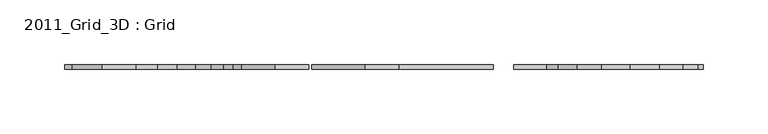
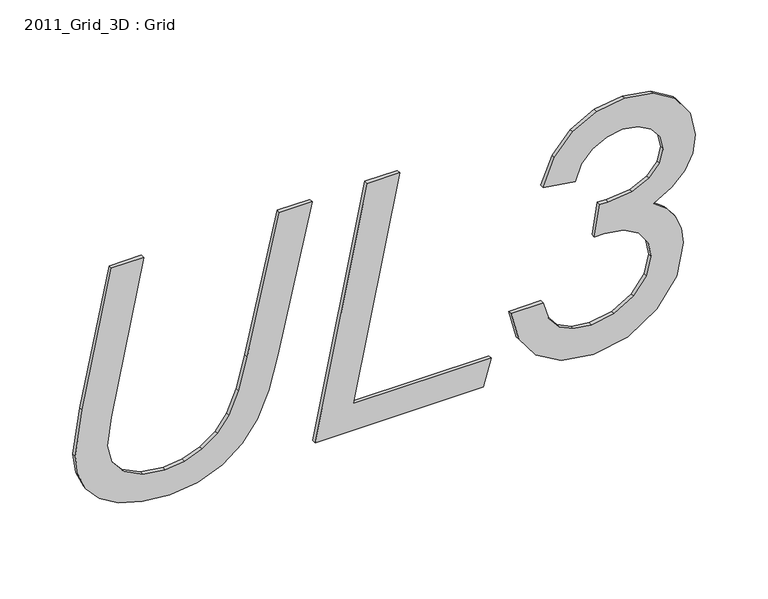
"""IFC4 building model written with IfcOpenShell, lengths in millimetres: proxy geometry, 2011_Grid_3D : Grid."""

import ifcopenshell
import ifcopenshell.guid

model = None  # the IFC model being written
_history = None  # IfcOwnerHistory: only IFC2X3 demands one
_inside = {}  # id of a spatial element -> (the spatial element, [elements in it])
_under = {}  # id of a project, library or spatial element -> (it, [spatial elements below it])
_declared = {}  # id of a project -> (the project, [libraries it declares])
_typed = {}  # id of a type object -> (the type object, [elements of that type])
_made_of = {}  # id of a material, layer set ... -> (it, [elements and type objects made of it])


def new_model(schema):
    """Start an empty IFC model of exactly this schema.

    Asked for "IFC4X3", IfcOpenShell would pick the latest addendum, in which some entities
    have other attributes; the version numbers below select the first issue.
    IFC2X3 requires an IfcOwnerHistory on every rooted entity: one is made here for all.
    """
    global model, _history
    if schema == "IFC4X3":
        model = ifcopenshell.file(schema_version=(4, 3, 0, 0))
    else:
        model = ifcopenshell.file(schema=schema)
    _inside.clear()
    _under.clear()
    _declared.clear()
    _typed.clear()
    _made_of.clear()
    _history = None
    if model.schema == "IFC2X3":
        org = make("IfcOrganization", Name="unknown")
        user = make(
            "IfcPersonAndOrganization",
            ThePerson=make("IfcPerson", FamilyName="unknown"),
            TheOrganization=org,
        )
        app = make(
            "IfcApplication",
            ApplicationDeveloper=org,
            Version="unknown",
            ApplicationFullName="unknown",
            ApplicationIdentifier="unknown",
        )
        _history = make(
            "IfcOwnerHistory",
            OwningUser=user,
            OwningApplication=app,
            ChangeAction="ADDED",
            CreationDate=0,
        )
    return model


def make(cls, **values):
    """One entity of the class cls with the attributes given. An attribute that is None is left unset."""
    return model.create_entity(
        cls, **{name: value for name, value in values.items() if value is not None}
    )


def rooted(cls, **values):
    """An entity with a GlobalId (a new one), such as an element, a storey or a relation."""
    return make(cls, GlobalId=ifcopenshell.guid.new(), OwnerHistory=_history, **values)


def si_unit(unit_type, name, prefix=None):
    """IfcSIUnit, for example si_unit("LENGTHUNIT", "METRE", prefix="MILLI")."""
    return make("IfcSIUnit", UnitType=unit_type, Prefix=prefix, Name=name)


def assignment(units):
    """IfcUnitAssignment: the units of a project."""
    return None if units is None else make("IfcUnitAssignment", Units=units)


def point(xyz):
    """IfcCartesianPoint."""
    return None if xyz is None else make("IfcCartesianPoint", Coordinates=xyz)


def direction(xyz):
    """IfcDirection."""
    return None if xyz is None else make("IfcDirection", DirectionRatios=xyz)


def frame(location, z_axis=None, x_axis=None):
    """IfcAxis2Placement3D, a coordinate frame: its origin and axes. An axis left out is left unset."""
    return make(
        "IfcAxis2Placement3D",
        Location=point(location),
        Axis=direction(z_axis),
        RefDirection=direction(x_axis),
    )


def origin():
    """The frame at (0, 0, 0) with its axes left unset."""
    return frame((0.0, 0.0, 0.0))


def place(relative_to, where):
    """IfcLocalPlacement: puts the frame where relative to a parent placement (None: the world)."""
    return make(
        "IfcLocalPlacement", PlacementRelTo=relative_to, RelativePlacement=where
    )


def context(
    kind, dimensions, precision=None, world=None, true_north=None, identifier=None
):
    """IfcGeometricRepresentationContext, for example the 3D "Model" context."""
    return make(
        "IfcGeometricRepresentationContext",
        ContextIdentifier=identifier,
        ContextType=kind,
        CoordinateSpaceDimension=dimensions,
        Precision=precision,
        WorldCoordinateSystem=world,
        TrueNorth=true_north,
    )


def project(units=None, contexts=None):
    """IfcProject with its units and contexts."""
    return rooted(
        "IfcProject",
        Name="project",
        RepresentationContexts=contexts,
        UnitsInContext=assignment(units),
    )


def spatial(cls, under=None, at=None, **own):
    """A site, building, storey or space (cls), placed at a placement, below another one or the project."""
    s = rooted(cls, ObjectPlacement=at, **own)
    if under is not None:
        _under.setdefault(under.id(), (under, []))[1].append(s)
    return s


def polyline(points):
    """IfcPolyline through the points."""
    return make("IfcPolyline", Points=[point(p) for p in points])


def outline(outer, holes=None, kind="AREA"):
    """IfcArbitraryClosedProfileDef: a profile drawn as a closed curve; with holes, ...WithVoids."""
    if holes is None:
        return make("IfcArbitraryClosedProfileDef", ProfileType=kind, OuterCurve=outer)
    return make(
        "IfcArbitraryProfileDefWithVoids",
        ProfileType=kind,
        OuterCurve=outer,
        InnerCurves=holes,
    )


def extrude(swept, where, along, depth):
    """IfcExtrudedAreaSolid: the profile swept, set in the frame where, extruded along a direction by depth."""
    return make(
        "IfcExtrudedAreaSolid",
        SweptArea=swept,
        Position=where,
        ExtrudedDirection=direction(along),
        Depth=depth,
    )


def shape(context_of_items, identifier, shape_type, items):
    """IfcShapeRepresentation: the items that make up one representation, for example the "Body"."""
    return make(
        "IfcShapeRepresentation",
        ContextOfItems=context_of_items,
        RepresentationIdentifier=identifier,
        RepresentationType=shape_type,
        Items=items,
    )


def source(mapping_origin, context_of_items, identifier, shape_type, items):
    """IfcRepresentationMap: a shape defined once, which mapped items show again and again."""
    return make(
        "IfcRepresentationMap",
        MappingOrigin=mapping_origin,
        MappedRepresentation=shape(context_of_items, identifier, shape_type, items),
    )


def transform(
    local_origin,
    x_axis=None,
    y_axis=None,
    z_axis=None,
    scale=None,
    scale2=None,
    scale3=None,
    uniform=True,
):
    """IfcCartesianTransformationOperator3D, or its non-uniform kind. x_axis, y_axis, z_axis: its Axis1, 2, 3."""
    if uniform:
        return make(
            "IfcCartesianTransformationOperator3D",
            Axis1=direction(x_axis),
            Axis2=direction(y_axis),
            LocalOrigin=point(local_origin),
            Scale=scale,
            Axis3=direction(z_axis),
        )
    return make(
        "IfcCartesianTransformationOperator3DnonUniform",
        Axis1=direction(x_axis),
        Axis2=direction(y_axis),
        LocalOrigin=point(local_origin),
        Scale=scale,
        Axis3=direction(z_axis),
        Scale2=scale2,
        Scale3=scale3,
    )


def mapped(mapping_source, mapping_target):
    """IfcMappedItem: shows the shape of a source again, moved by a transform."""
    return make(
        "IfcMappedItem", MappingSource=mapping_source, MappingTarget=mapping_target
    )


def made_of(thing, what):
    """Note that an element or type object is made of a material, layer set ...; save() writes the relation."""
    if what is not None:
        _made_of.setdefault(what.id(), (what, []))[1].append(thing)
    return thing


def element(
    cls,
    number,
    at=None,
    inside=None,
    cuts=None,
    type_object=None,
    material=None,
    context=None,
    identifier="Body",
    shape_type=None,
    held_by="IfcProductDefinitionShape",
    body=None,
    shapes=None,
    **own,
):
    """One element of the class cls, such as IfcWall. Its Tag is "e" and its number.

    at: its placement. inside: the storey or other place that contains it. cuts: it is an
    opening in that element (IfcRelVoidsElement). A single representation is given by context,
    identifier, shape_type and body (its items); several are given by shapes. held_by: the class
    of the entity that holds the representations. save() writes the other relations.
    """
    e = rooted(cls, Tag="e%d" % number, ObjectPlacement=at, **own)
    if body is not None:
        shapes = [shape(context, identifier, shape_type, body)]
    if shapes is not None:
        e.Representation = make(held_by, Representations=shapes)
    if inside is not None:
        _inside.setdefault(inside.id(), (inside, []))[1].append(e)
    if cuts is not None:
        rooted(
            "IfcRelVoidsElement", RelatingBuildingElement=cuts, RelatedOpeningElement=e
        )
    if type_object is not None:
        _typed.setdefault(type_object.id(), (type_object, []))[1].append(e)
    return made_of(e, material)


def aggregate(whole, parts):
    """IfcRelAggregates: a whole, such as a stair, and the parts it consists of."""
    return rooted("IfcRelAggregates", RelatingObject=whole, RelatedObjects=parts)


def save(model, path):
    """Write the relations noted so far, then the file.

    IfcRelAggregates (storeys below a building ...), IfcRelContainedInSpatialStructure (elements
    in a storey), IfcRelDefinesByType, IfcRelAssociatesMaterial and IfcRelDeclares: one each for
    every whole, place, type object, material and project.
    """
    for whole, parts in _under.values():
        aggregate(whole, parts)
    for where, things in _inside.values():
        rooted(
            "IfcRelContainedInSpatialStructure",
            RelatedElements=things,
            RelatingStructure=where,
        )
    for kind, things in _typed.values():
        rooted("IfcRelDefinesByType", RelatedObjects=things, RelatingType=kind)
    for what, things in _made_of.values():
        rooted("IfcRelAssociatesMaterial", RelatedObjects=things, RelatingMaterial=what)
    for by, libraries in _declared.values():
        rooted("IfcRelDeclares", RelatingContext=by, RelatedDefinitions=libraries)
    model.write(path)


def proxy_2011_grid_3d_grid_08464130(model_context):
    return source(origin(), model_context, "Body", "SweptSolid", [
        extrude(outline(polyline([(101.4447294, 47277.8299768), (-9.5457855, 47254.7296731), (-46.3278141, 47249.0785258), (-62.2836301, 47251.2224918), (-76.4424804, 47257.6543897), (-88.2714718, 47268.3866123), (-97.2377109, 47283.4315526), (-102.8888581, 47302.2191386), (-104.7725739, 47324.1792986), (-102.1081075, 47346.374923), (-94.1147085, 47365.6706165), (-81.7032524, 47381.5706646), (-65.784615, 47393.5793525), (-44.9584024, 47402.6757168), (-17.8242205, 47409.8387938), (101.4447294, 47437.0039577), (101.4447294, 47411.0780804), (-10.7355007, 47385.4992034), (-36.7791103, 47378.8070553), (-54.6310349, 47371.3217638), (-66.7202764, 47362.0271137), (-75.4758368, 47349.90689), (-80.7923767, 47335.8285933), (-82.5645566, 47320.6597244), (-80.0983761, 47302.5599424), (-72.6998347, 47287.8186274), (-61.2488258, 47278.0220662), (-46.6252429, 47274.7565458), (-23.5745107, 47277.8795482), (101.4447294, 47303.5575682), (101.4447294, 47277.8299768)])), frame((0.0, -3.175, 0.0), z_axis=(0.0, 1.0, 0.0), x_axis=(0.0, 0.0, 1.0)), (0.0, 0.0, 1.0), 3.175),
        extrude(outline(polyline([(-101.6, 47439.4329596), (-101.6, 47572.6810633), (-79.3919827, 47579.0262111), (-79.3919827, 47469.7211261), (101.4447294, 47506.4535832), (101.4447294, 47480.6764203), (-101.6, 47439.4329596)])), frame((0.0, -3.175, 0.0), z_axis=(0.0, 1.0, 0.0), x_axis=(0.0, 0.0, 1.0)), (0.0, 0.0, 1.0), 3.175),
        extrude(outline(polyline([(-47.6662438, 47594.8890806), (-71.0391905, 47600.7385137), (-89.2071332, 47614.3210957), (-100.8812137, 47634.4966828), (-104.7725739, 47660.1251313), (-99.641927, 47687.271706), (-84.2499865, 47710.3162418), (-61.8684691, 47726.061379), (-35.7690916, 47731.3097581), (-23.320457, 47729.8473998), (-12.3465734, 47725.460325), (-2.8598339, 47718.0989621), (5.1273687, 47707.7137398), (13.6970361, 47722.2939475), (24.2371693, 47732.623402), (36.7477683, 47738.7764604), (51.2288332, 47740.8274798), (70.7352055, 47736.9547089), (86.9202895, 47725.3363963), (97.8136194, 47707.4720789), (101.4447294, 47684.8612934), (98.0428874, 47662.709044), (87.8373617, 47643.7417614), (71.4106167, 47629.1863394), (49.3451174, 47620.2696717), (45.2306856, 47645.6502629), (58.2865708, 47650.570231), (68.0087748, 47659.2824164), (74.0502974, 47670.5475323), (76.0641382, 47683.1262921), (74.0936724, 47695.6554804), (68.1822749, 47706.0778813), (59.3833395, 47713.1046368), (48.7502598, 47715.4468886), (37.1877151, 47712.6894758), (27.5832433, 47704.4172372), (21.1141669, 47690.803673), (18.9578081, 47672.0222834), (19.4039513, 47665.1318495), (-6.4227831, 47660.8687033), (-6.4227831, 47668.8497095), (-8.6968742, 47684.0805428), (-15.5191473, 47695.8661591), (-25.8362089, 47703.413415), (-38.5946653, 47705.9291669), (-53.7015699, 47702.4343785), (-66.9991159, 47691.9500132), (-76.293766, 47676.6572156), (-79.3919827, 47658.7371302), (-77.551642, 47644.3118333), (-72.0306199, 47632.9599673), (-62.2588444, 47624.8798182), (-47.6662438, 47620.2696717), (-47.6662438, 47594.8890806)])), frame((0.0, -3.175, 0.0), z_axis=(0.0, 1.0, 0.0), x_axis=(0.0, 0.0, 1.0)), (0.0, 0.0, 1.0), 3.175),
    ])


if __name__ == "__main__":
    model = new_model("IFC4")
    model_context = context("Model", 3, world=origin())
    ifc_project = project(units=[si_unit("LENGTHUNIT", "METRE", prefix="MILLI")], contexts=[model_context])
    site = spatial("IfcSite", under=ifc_project)
    building = spatial("IfcBuilding", under=site)
    placement = place(None, origin())
    proxy_2011_grid_3d_grid_shape = proxy_2011_grid_3d_grid_08464130(model_context)
    element("IfcBuildingElementProxy", 1, Name="2011_Grid_3D : Grid", ObjectType="2011_Grid_3D : Grid", at=placement, inside=building, context=model_context, shape_type="MappedRepresentation", body=[
        mapped(proxy_2011_grid_3d_grid_shape, transform((0.0, 0.0, 0.0), x_axis=(1.0, 0.0, 0.0), y_axis=(0.0, 1.0, 0.0), z_axis=(0.0, 0.0, 1.0))),
    ])
    save(model, "model.ifc")

# Revit data of these elements
# Type "2011_Grid_3D : Grid"
#   Workplane [instance default] = "LEVEL"
#   Grid [instance default] = "S"
#   t [instance default] = 12' - 6"
#   built-in parameter 1001306 [instance default] = 50 (stored number, unit not read)
#   d [instance default] = 2
#   Symbol At End 2 [instance default] = yes
#   Symbol At End 1 [instance default] = yes
#   Robust [instance default] = yes
#   No of grid markers [instance default] = 3
#   Grid Height Visible = yes
#   Height = 0
#   Assembly Code = ""
# Element 1 (IfcBuildingElementProxy, "2011_Grid_3D : Grid")
#   Workplane = "UL3"
#   Grid = "A"
#   t = 11' - 0.37148"
#   built-in parameter 1001306 = 154.433 (stored number, unit not read)
#   d = 7
#   Robust = no
#   No of grid markers = 8
#   Materials on its faces: "Letter"
# Materials
#   "Letter": class "Unassigned", colour RGB 178 187 30, transparency 0, Comments = "Rendering appearance not upgraded "
